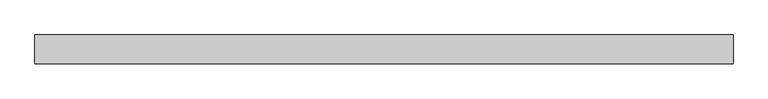
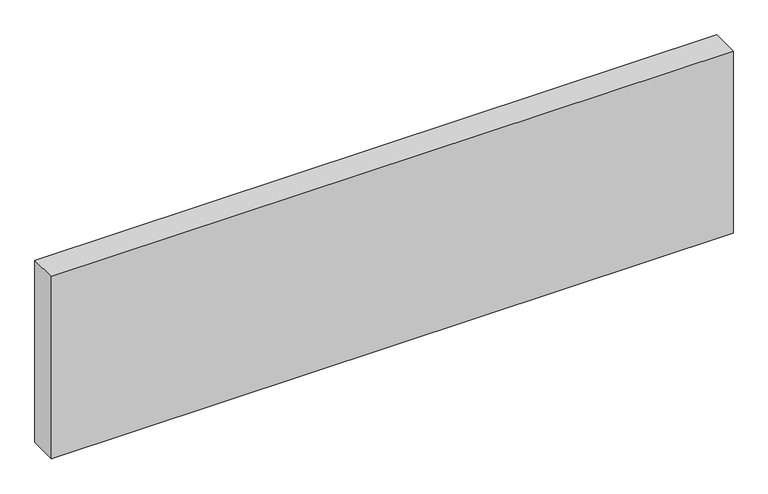
"""IFC4 building model written with IfcOpenShell, lengths in millimetres: proxy geometry, Generic Models 7:Generic Models 1:6:Generic Models 1:6 : Generic Models 7:Generic Models 1:337419:5 : Generic Models 7:Generic Models 1:6:Generic Models 1:6 : Generic Models 7:Generic Models 1:337419:312901."""

from ifc_helpers import new_model, si_unit, origin, place, context, project, spatial, faceted_brep, source, transform, mapped, element, save


def generic_models_b96f1b28(model_context):
    return source(origin(), model_context, "Body", "Brep", [
        faceted_brep([(596182.8367242, -536557.2913358, 0.0), (596182.8367242, -536760.4913358, 0.0), (596182.8367242, -536760.4913358, -1377.3372439), (596182.8367242, -536557.2913358, -1377.3372439), (591306.0367242, -536557.2913358, 0.0), (591306.0367242, -536557.2913358, -127.0), (591306.0367242, -536557.2913358, -1377.3372439), (591306.0367242, -536760.4913358, -1377.3372439), (591306.0367242, -536760.4913358, 0.0)], [[[0, 1, 2, 3]], [[4, 5, 6, 7, 8]], [[0, 3, 6, 5, 4]], [[3, 2, 7, 6]], [[2, 1, 8, 7]], [[1, 0, 4, 8]]]),
    ])


if __name__ == "__main__":
    model = new_model("IFC4")
    model_context = context("Model", 3, world=origin())
    ifc_project = project(units=[si_unit("LENGTHUNIT", "METRE", prefix="MILLI")], contexts=[model_context])
    site = spatial("IfcSite", under=ifc_project)
    building = spatial("IfcBuilding", under=site)
    placement = place(None, origin())
    generic_models_shape = generic_models_b96f1b28(model_context)
    element("IfcBuildingElementProxy", 1, Name="Generic Models 7:Generic Models 1:6:Generic Models 1:6 : Generic Models 7:Generic Models 1:337419:5 : Generic Models 7:Generic Models 1:6:Generic Models 1:6 : Generic Models 7:Generic Models 1:337419:312901", ObjectType="Generic Models 7:Generic Models 1:6:Generic Models 1:6 : Generic Models 7:Generic Models 1:337419:5 : Generic Models 7:Generic Models 1:6:Generic Models 1:6 : Generic Models 7:Generic Models 1:337419:312901", at=placement, inside=building, context=model_context, shape_type="MappedRepresentation", body=[
        mapped(generic_models_shape, transform((0.0, 0.0, 0.0), x_axis=(1.0, 0.0, 0.0), y_axis=(0.0, 1.0, 0.0), z_axis=(0.0, 0.0, 1.0))),
    ])
    save(model, "model.ifc")

# Revit data of these elements
# Type "Generic Models 7:Generic Models 1:6:Generic Models 1:6 : Generic Models 7:Generic Models 1:337419:5 : Generic Models 7:Generic Models 1:6:Generic Models 1:6 : Generic Models 7:Generic Models 1:337419:312901"
#   NameOverride = "Generic Models 7:Generic Models 1:6:Generic Models 1:6 : Generic Models 7:Generic Models 1:337419:312901"
#   ObjectTypeOverride = "Generic Models 1:6 : Generic Models 7:Generic Models 1:337419"
#   Reference = "Generic Models 1"
#   Tag = "312901"
# Element 1 (IfcBuildingElementProxy, "Generic Models 7:Generic Models 1:6:Generic Models 1:6 : Generic Models 7:Generic Models 1:337419:5 : Generic Models 7:Generic Models 1:6:Generic Models 1:6 : Generic Models 7:Generic Models 1:337419:312901")
#   Materials on its faces: "CONCRETE FROST WALL - SEE STRUCT DWGS."
# Materials
#   "CONCRETE FROST WALL - SEE STRUCT DWGS.": class "Concrete", colour RGB 115 116 108, transparency 0, Description = "Lightweight concrete", Cost = 0
